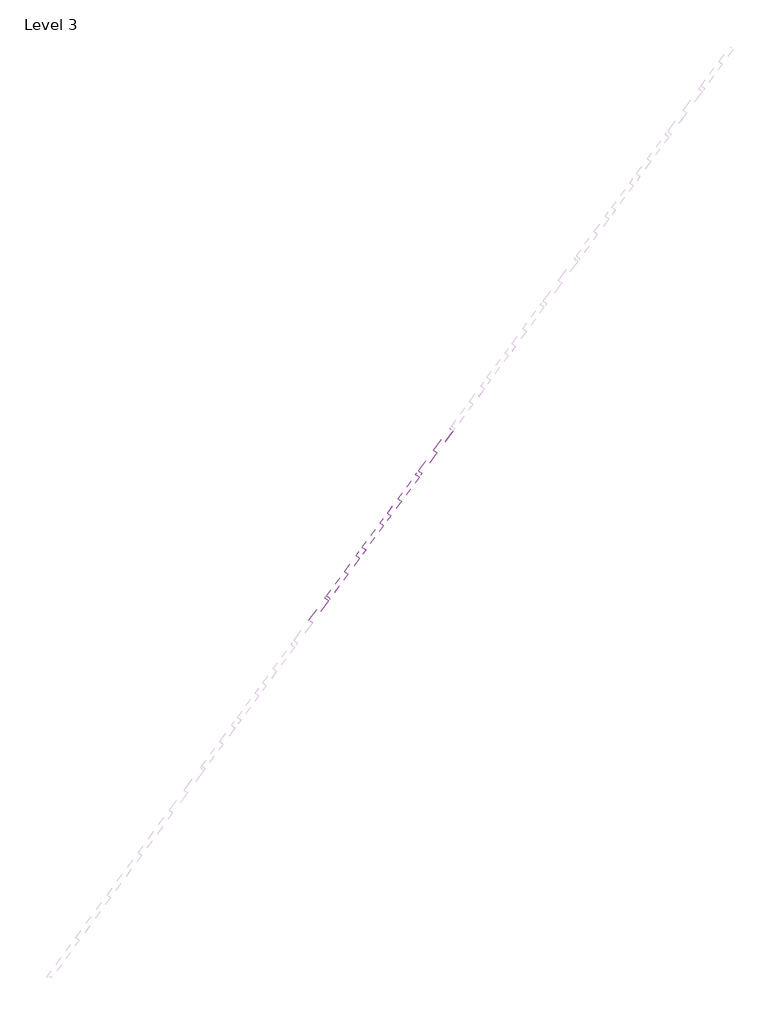
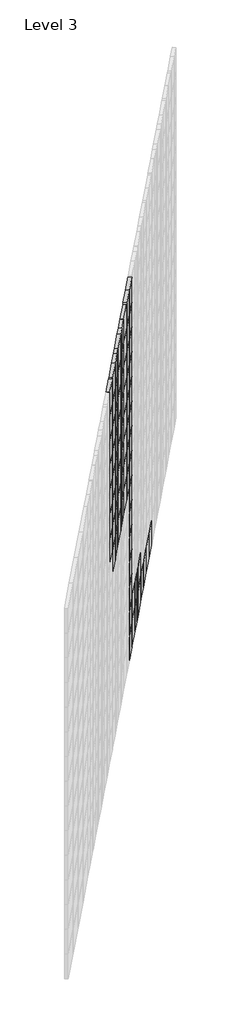
# One storey, part 6 of 9: 117 plates.
# Revit data of these elements (continued)
# Elements 1, 2, 3, 4, 5, 6, 7, 8, 9, 10, 11, 12, 13, 14, 15, 16, 17, 18, 19, 20, 21, 22, 23, 24, 25, 26, 27, 28, 29, 30, 31, 32, 33, 34, 35, 36, 37, 38, 39, 40, 41, 42, 43, 44, 45, 46, 47, 48, 49, 50, 51, 52, 53, 54, 55, 56, 57, 58, 59, 60, 61, 62, 63, 64, 65, 66, 67, 68, 69, 70, 71, 72, 73, 74, 75, 76, 77, 78, 79, 80, 81, 82, 83, 84, 85, 86, 87, 88, 89, 90, 91, 92, 93, 94, 95, 96, 97, 98, 99, 100, 101, 102, 103, 104, 105, 106, 107, 108, 109, 110, 111, 112, 113, 114, 115, 116, 117 (IfcPlate, "System Panel : Glazed") (continued)
#   Phase Created = New Construction
#   Materials on its faces: "Glass"
# Materials
#   "Glass": class "Glass", colour RGB 218 227 224, transparency 0.85, Description = "Soda Lime Glass", Cost = 0
